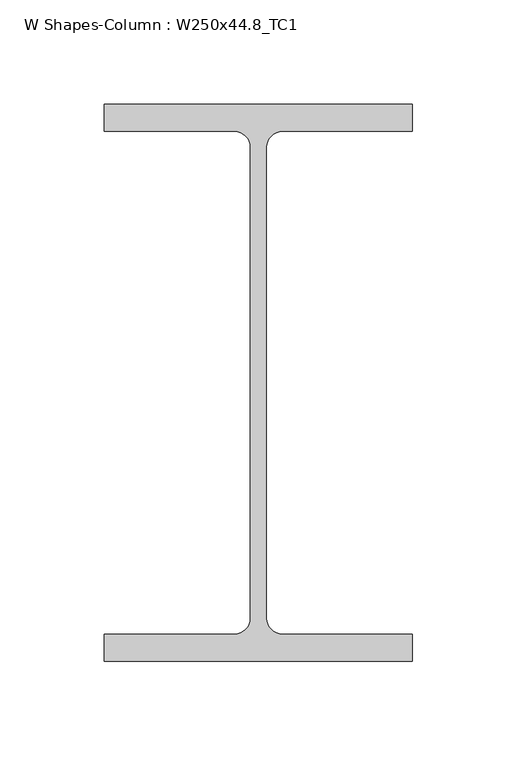
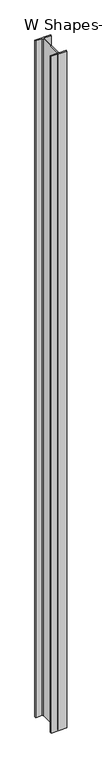
"""IFC4 building model written with IfcOpenShell, lengths in millimetres: column geometry, W Shapes-Column : W250x44.8_TC1."""

from ifc_helpers import new_model, si_unit, point, frame, frame_2d, origin, place, context, project, spatial, polyline, circle_curve, trimmed, segment, composite_curve, outline, extrude, source, transform, mapped, element, save


def w_shapes_column_w250x44_8_tc1_79b3104d(model_context):
    return source(origin(), model_context, "Body", "SweptSolid", [
        extrude(outline(composite_curve([segment(polyline([(73.787, 133.35), (73.787, 120.396), (11.43, 120.396)]), True, "CONTINUOUS"), segment(trimmed(circle_curve(frame_2d((11.43, 112.776)), 7.62), [point((11.43, 120.396))], [point((3.81, 112.776))], True, "CARTESIAN"), True, "CONTINUOUS"), segment(polyline([(3.81, 112.776), (3.81, -112.776)]), True, "CONTINUOUS"), segment(trimmed(circle_curve(frame_2d((11.43, -112.776)), 7.62), [point((3.81, -112.776))], [point((11.43, -120.396))], True, "CARTESIAN"), True, "CONTINUOUS"), segment(polyline([(11.43, -120.396), (73.787, -120.396), (73.787, -133.35), (-73.787, -133.35), (-73.787, -120.396), (-11.43, -120.396)]), True, "CONTINUOUS"), segment(trimmed(circle_curve(frame_2d((-11.43, -112.776)), 7.62), [point((-11.43, -120.396))], [point((-3.81, -112.776))], True, "CARTESIAN"), True, "CONTINUOUS"), segment(polyline([(-3.81, -112.776), (-3.81, 112.776)]), True, "CONTINUOUS"), segment(trimmed(circle_curve(frame_2d((-11.43, 112.776)), 7.62), [point((-3.81, 112.776))], [point((-11.43, 120.396))], True, "CARTESIAN"), True, "CONTINUOUS"), segment(polyline([(-11.43, 120.396), (-73.787, 120.396), (-73.787, 133.35), (73.787, 133.35)]), True, "CONTINUOUS")], self_intersect=False)), frame((0.0, 0.0, 200.0), z_axis=(0.0, 0.0, 1.0), x_axis=(1.0, 0.0, 0.0)), (0.0, 0.0, 1.0), 6750.0),
    ])


if __name__ == "__main__":
    model = new_model("IFC4")
    model_context = context("Model", 3, world=origin())
    ifc_project = project(units=[si_unit("LENGTHUNIT", "METRE", prefix="MILLI")], contexts=[model_context])
    site = spatial("IfcSite", under=ifc_project)
    building = spatial("IfcBuilding", under=site)
    placement = place(None, origin())
    w_shapes_column_w250x44_8_tc1_shape = w_shapes_column_w250x44_8_tc1_79b3104d(model_context)
    element("IfcColumn", 1, ObjectType="W Shapes-Column : W250x44.8_TC1", at=placement, inside=building, context=model_context, shape_type="MappedRepresentation", body=[
        mapped(w_shapes_column_w250x44_8_tc1_shape, transform((0.0, 0.0, 0.0), x_axis=(1.0, 0.0, 0.0), y_axis=(0.0, 1.0, 0.0), z_axis=(0.0, 0.0, 1.0))),
    ])
    save(model, "model.ifc")

# Revit data of these elements
# Type "W Shapes-Column : W250x44.8_TC1"
#   Section Name Key = "W10X30"
#   Assembly Code = "B10"
#   Width = 14.7574 cm
#   Web Thickness = 0.762 cm
#   Web Fillet = 0.762 cm
#   Warping Constant = 111173.8 cm⁶
#   Torsional Moment of Inertia = 25.8896 cm⁴
#   Section Area = 57.0321 cm²
#   Plastic Modulus weak axis = 144.862 cm³
#   Plastic Modulus strong axis = 599.767 cm³
#   Perimeter = 1.09454 m²/m
#   Nominal Weight = 44.6449 kgf/m
#   Moment of Inertia weak axis = 695.106 cm⁴
#   Moment of Inertia strong axis = 7075.93 cm⁴
#   Height = 26.67 cm
#   Flange Thickness = 1.2954 cm
#   Elastic Modulus weak axis = 94.2256 cm³
#   Elastic Modulus strong axis = 530.941 cm³
#   Clear Web Height = 20.955 cm
#   Centroid Vertical = 13.335 cm
#   Centroid Horizontal = 7.3787 cm
#   Bolt Spacing = 6.985 cm
#   Structural Material [instance default] = Steel ASTM A992
#   Principal Axes Angle = 0
# Element 1 (IfcColumn, "W Shapes-Column : W250x44.8_TC1")
#   Structural Material = none
# Materials
#   "Steel ASTM A992": class "Metal", colour RGB 199 199 199, transparency 0, Description = "Structural steel 50ksi", Cost = 0
